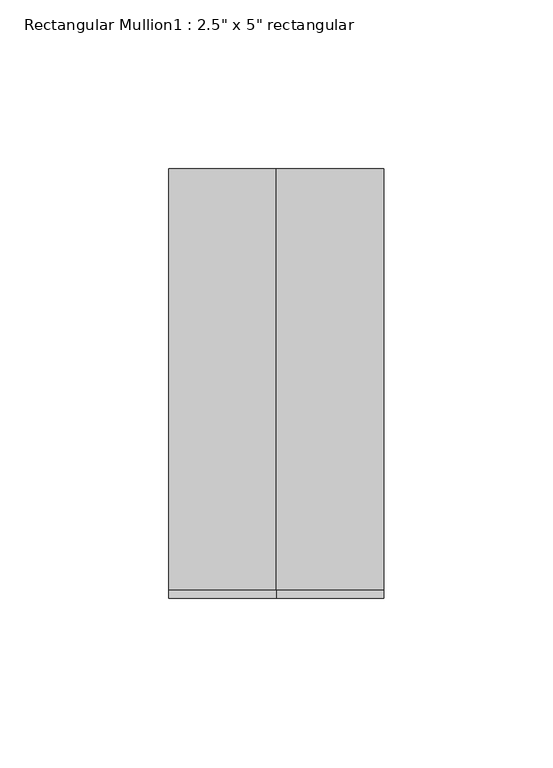
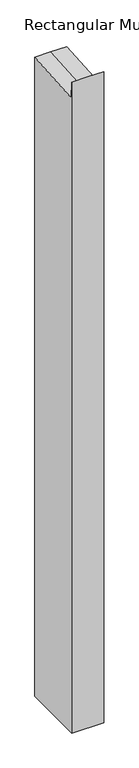
"""IFC4 building model written with IfcOpenShell, lengths in millimetres: member geometry."""

from ifc_helpers import new_model, si_unit, origin, place, context, project, spatial, faceted_brep, source, transform, mapped, element, save


def member_23db0025(model_context):
    return source(origin(), model_context, "Body", "Brep", [
        faceted_brep([(31.75, 63.5, -1339.4207165), (31.75, -63.5, -1339.4207165), (-31.75, -63.5, -1339.4207165), (-31.75, 63.5, -1339.4207165), (-31.75, 63.5, 4.6293267), (0.0, 63.5, 4.6293267), (31.75, 63.5, 4.6293267), (-31.75, -63.5, 29.3948455), (-31.75, -60.9736199, -4.616608), (31.75, -63.5, 29.3948455), (0.0, -63.5, 29.3948455), (31.75, -60.9736199, -4.616608), (0.0, -60.9736199, -4.616608)], [[[0, 1, 2, 3]], [[4, 5, 6, 0, 3]], [[7, 8, 4, 3, 2]], [[9, 10, 7, 2, 1]], [[6, 11, 9, 1, 0]], [[6, 5, 12, 11]], [[5, 4, 8, 12]], [[8, 7, 10, 12]], [[10, 9, 11, 12]]]),
    ])


if __name__ == "__main__":
    model = new_model("IFC4")
    model_context = context("Model", 3, world=origin())
    ifc_project = project(units=[si_unit("LENGTHUNIT", "METRE", prefix="MILLI")], contexts=[model_context])
    site = spatial("IfcSite", under=ifc_project)
    building = spatial("IfcBuilding", under=site)
    placement = place(None, origin())
    member_shape = member_23db0025(model_context)
    element("IfcMember", 1, ObjectType="Rectangular Mullion1 : 2.5\" x 5\" rectangular", at=placement, inside=building, context=model_context, shape_type="MappedRepresentation", body=[
        mapped(member_shape, transform((0.0, 0.0, 0.0), x_axis=(1.0, 0.0, 0.0), y_axis=(0.0, 1.0, 0.0), z_axis=(0.0, 0.0, 1.0))),
    ])
    save(model, "model.ifc")

# Revit data of these elements
# Type "Rectangular Mullion1 : 2.5\" x 5\" rectangular"
#   built-in parameter 1007304 = 0.416667 (stored number, unit not read)
#   built-in parameter 1007301 = 0.104167 (stored number, unit not read)
#   built-in parameter 1007300 = 0.104167 (stored number, unit not read)
# Element 1 (IfcMember, "Rectangular Mullion1 : 2.5\" x 5\" rectangular")
#   Materials on its faces: "support-frame"
# Materials
#   "support-frame": class "Unassigned", colour RGB 233 233 233, transparency 0, Cost = 0
